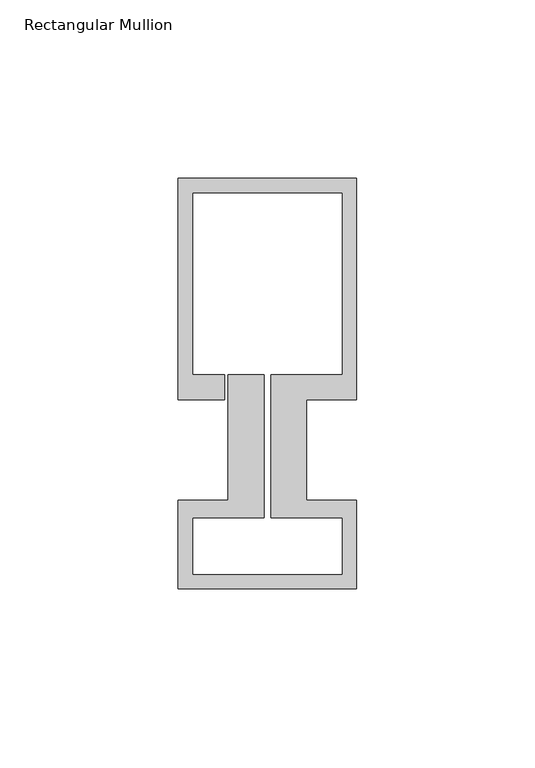
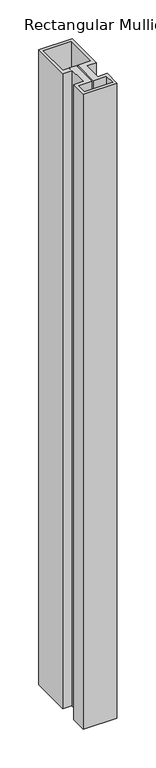
"""IFC4 building model written with IfcOpenShell, lengths in millimetres: member geometry, Rectangular Mullion : Schueco_FWS-50-HI_Tran_CovCap-20mm_Tran-55mm."""

from ifc_helpers import new_model, si_unit, frame, origin, place, context, project, spatial, polyline, outline, extrude, source, transform, mapped, element, save


def rectangular_mullion_9c86bac1(model_context):
    return source(origin(), model_context, "Body", "SweptSolid", [
        extrude(outline(polyline([(0.0, 90.0), (0.0, 28.0), (-14.0, 28.0), (-14.0, -0.1), (0.0, -0.1), (0.0, -25.0), (-50.0, -25.0), (-50.0, -0.1), (-36.0, -0.1), (-36.0, 35.0), (-26.0, 35.0), (-26.0, -5.0), (-46.0, -5.0), (-46.0, -21.0), (-4.0, -21.0), (-4.0, -5.0), (-24.0, -5.0), (-24.0, 35.0), (-4.0, 35.0), (-4.0, 86.0), (-46.0, 86.0), (-46.0, 35.0), (-37.0, 35.0), (-37.0, 28.0), (-50.0, 28.0), (-50.0, 90.0), (0.0, 90.0)])), frame((0.0, 0.0, -1000.0), z_axis=(0.0, 0.0, 1.0), x_axis=(1.0, 0.0, 0.0)), (0.0, 0.0, 1.0), 1000.0),
    ])


if __name__ == "__main__":
    model = new_model("IFC4")
    model_context = context("Model", 3, world=origin())
    ifc_project = project(units=[si_unit("LENGTHUNIT", "METRE", prefix="MILLI")], contexts=[model_context])
    site = spatial("IfcSite", under=ifc_project)
    building = spatial("IfcBuilding", under=site)
    placement = place(None, origin())
    rectangular_mullion_shape = rectangular_mullion_9c86bac1(model_context)
    element("IfcMember", 1, ObjectType="Rectangular Mullion : Schueco_FWS-50-HI_Tran_CovCap-20mm_Tran-55mm", at=placement, inside=building, context=model_context, shape_type="MappedRepresentation", body=[
        mapped(rectangular_mullion_shape, transform((0.0, 0.0, 0.0), x_axis=(1.0, 0.0, 0.0), y_axis=(0.0, 1.0, 0.0), z_axis=(0.0, 0.0, 1.0))),
    ])
    save(model, "model.ifc")

# Revit data of these elements
# Type "Rectangular Mullion : Schueco_FWS-50-HI_Tran_CovCap-20mm_Tran-55mm"
#   Model = "FWS 50.HI"
#   Manufacturer = "Schueco International KG"
#   Type Comments = "Transom"
#   Schueco thermal insulation standard = "Highly thermally insulated"
#   Burglar resistance = "RC 3"
#   Thermal insulation = "to 0.90 W/(m²K)"
#   built-in parameter 1007322 = 0.377297 (stored number, unit not read)
#   built-in parameter 1007321 = 0.0360892 (stored number, unit not read)
#   built-in parameter 1007320 = 0.0360892 (stored number, unit not read)
# Element 1 (IfcMember, "Rectangular Mullion : Schueco_FWS-50-HI_Tran_CovCap-20mm_Tran-55mm")
#   Materials on its faces: "Alu"
# Materials
#   "Alu": class "Glas", colour RGB 140 140 140, transparency 0
